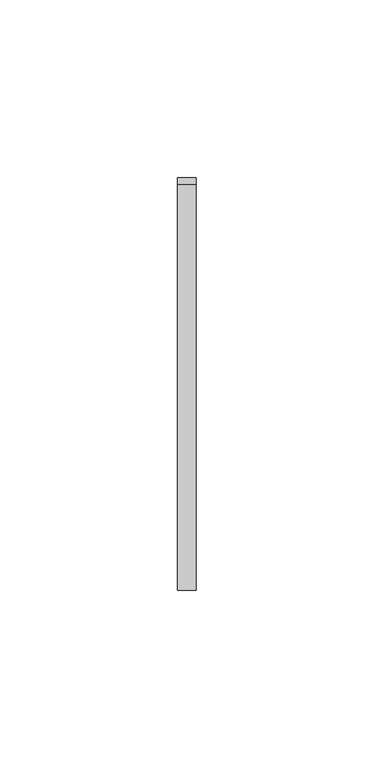
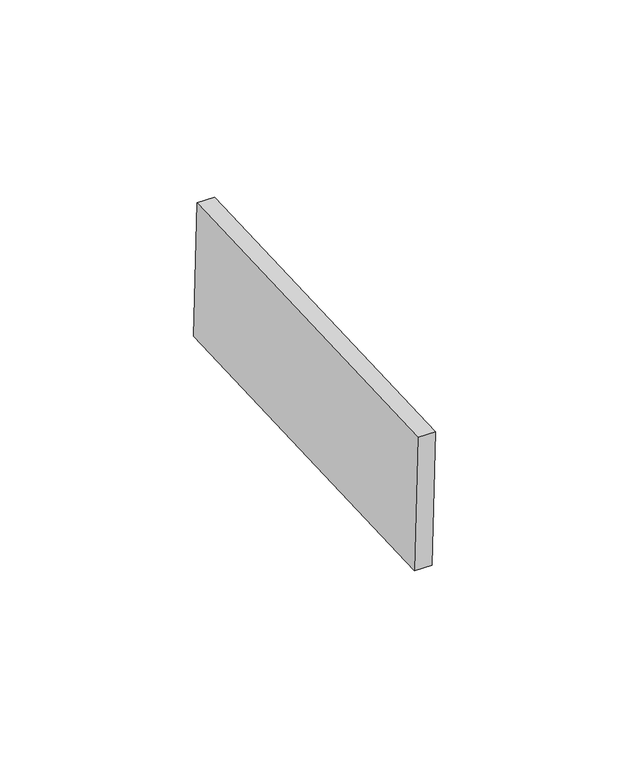
"""IFC4 building model written with IfcOpenShell, lengths in millimetres: proxy geometry, Inner panel:Inner panel:1:Inner panel:1 : Inner panel:Inner panel:300324:2:Inner panel:1:Inner panel:1 : Inner panel:Inner panel:300324:2 : Inner panel:Inner panel:1:Inner panel:1 : Inner panel:Inner panel:300324:300043:100 : Inner panel:Inner panel:1:Inner panel:1 : Inner panel:Inner panel:300324:2:Inner panel:1:Inner panel:1 : Inner panel:Inner panel:300324:2 : Inner panel:Inner panel:1:Inner panel:1 : Inner panel:Inner panel:300324:300043:308120."""

import ifcopenshell
import ifcopenshell.guid

model = None  # the IFC model being written
_history = None  # IfcOwnerHistory: only IFC2X3 demands one
_inside = {}  # id of a spatial element -> (the spatial element, [elements in it])
_under = {}  # id of a project, library or spatial element -> (it, [spatial elements below it])
_declared = {}  # id of a project -> (the project, [libraries it declares])
_typed = {}  # id of a type object -> (the type object, [elements of that type])
_made_of = {}  # id of a material, layer set ... -> (it, [elements and type objects made of it])


def new_model(schema):
    """Start an empty IFC model of exactly this schema.

    Asked for "IFC4X3", IfcOpenShell would pick the latest addendum, in which some entities
    have other attributes; the version numbers below select the first issue.
    IFC2X3 requires an IfcOwnerHistory on every rooted entity: one is made here for all.
    """
    global model, _history
    if schema == "IFC4X3":
        model = ifcopenshell.file(schema_version=(4, 3, 0, 0))
    else:
        model = ifcopenshell.file(schema=schema)
    _inside.clear()
    _under.clear()
    _declared.clear()
    _typed.clear()
    _made_of.clear()
    _history = None
    if model.schema == "IFC2X3":
        org = make("IfcOrganization", Name="unknown")
        user = make(
            "IfcPersonAndOrganization",
            ThePerson=make("IfcPerson", FamilyName="unknown"),
            TheOrganization=org,
        )
        app = make(
            "IfcApplication",
            ApplicationDeveloper=org,
            Version="unknown",
            ApplicationFullName="unknown",
            ApplicationIdentifier="unknown",
        )
        _history = make(
            "IfcOwnerHistory",
            OwningUser=user,
            OwningApplication=app,
            ChangeAction="ADDED",
            CreationDate=0,
        )
    return model


def make(cls, **values):
    """One entity of the class cls with the attributes given. An attribute that is None is left unset."""
    return model.create_entity(
        cls, **{name: value for name, value in values.items() if value is not None}
    )


def rooted(cls, **values):
    """An entity with a GlobalId (a new one), such as an element, a storey or a relation."""
    return make(cls, GlobalId=ifcopenshell.guid.new(), OwnerHistory=_history, **values)


def si_unit(unit_type, name, prefix=None):
    """IfcSIUnit, for example si_unit("LENGTHUNIT", "METRE", prefix="MILLI")."""
    return make("IfcSIUnit", UnitType=unit_type, Prefix=prefix, Name=name)


def assignment(units):
    """IfcUnitAssignment: the units of a project."""
    return None if units is None else make("IfcUnitAssignment", Units=units)


def point(xyz):
    """IfcCartesianPoint."""
    return None if xyz is None else make("IfcCartesianPoint", Coordinates=xyz)


def direction(xyz):
    """IfcDirection."""
    return None if xyz is None else make("IfcDirection", DirectionRatios=xyz)


def frame(location, z_axis=None, x_axis=None):
    """IfcAxis2Placement3D, a coordinate frame: its origin and axes. An axis left out is left unset."""
    return make(
        "IfcAxis2Placement3D",
        Location=point(location),
        Axis=direction(z_axis),
        RefDirection=direction(x_axis),
    )


def origin():
    """The frame at (0, 0, 0) with its axes left unset."""
    return frame((0.0, 0.0, 0.0))


def place(relative_to, where):
    """IfcLocalPlacement: puts the frame where relative to a parent placement (None: the world)."""
    return make(
        "IfcLocalPlacement", PlacementRelTo=relative_to, RelativePlacement=where
    )


def context(
    kind, dimensions, precision=None, world=None, true_north=None, identifier=None
):
    """IfcGeometricRepresentationContext, for example the 3D "Model" context."""
    return make(
        "IfcGeometricRepresentationContext",
        ContextIdentifier=identifier,
        ContextType=kind,
        CoordinateSpaceDimension=dimensions,
        Precision=precision,
        WorldCoordinateSystem=world,
        TrueNorth=true_north,
    )


def project(units=None, contexts=None):
    """IfcProject with its units and contexts."""
    return rooted(
        "IfcProject",
        Name="project",
        RepresentationContexts=contexts,
        UnitsInContext=assignment(units),
    )


def spatial(cls, under=None, at=None, **own):
    """A site, building, storey or space (cls), placed at a placement, below another one or the project."""
    s = rooted(cls, ObjectPlacement=at, **own)
    if under is not None:
        _under.setdefault(under.id(), (under, []))[1].append(s)
    return s


def polyline(points):
    """IfcPolyline through the points."""
    return make("IfcPolyline", Points=[point(p) for p in points])


def outline(outer, holes=None, kind="AREA"):
    """IfcArbitraryClosedProfileDef: a profile drawn as a closed curve; with holes, ...WithVoids."""
    if holes is None:
        return make("IfcArbitraryClosedProfileDef", ProfileType=kind, OuterCurve=outer)
    return make(
        "IfcArbitraryProfileDefWithVoids",
        ProfileType=kind,
        OuterCurve=outer,
        InnerCurves=holes,
    )


def extrude(swept, where, along, depth):
    """IfcExtrudedAreaSolid: the profile swept, set in the frame where, extruded along a direction by depth."""
    return make(
        "IfcExtrudedAreaSolid",
        SweptArea=swept,
        Position=where,
        ExtrudedDirection=direction(along),
        Depth=depth,
    )


def shape(context_of_items, identifier, shape_type, items):
    """IfcShapeRepresentation: the items that make up one representation, for example the "Body"."""
    return make(
        "IfcShapeRepresentation",
        ContextOfItems=context_of_items,
        RepresentationIdentifier=identifier,
        RepresentationType=shape_type,
        Items=items,
    )


def source(mapping_origin, context_of_items, identifier, shape_type, items):
    """IfcRepresentationMap: a shape defined once, which mapped items show again and again."""
    return make(
        "IfcRepresentationMap",
        MappingOrigin=mapping_origin,
        MappedRepresentation=shape(context_of_items, identifier, shape_type, items),
    )


def transform(
    local_origin,
    x_axis=None,
    y_axis=None,
    z_axis=None,
    scale=None,
    scale2=None,
    scale3=None,
    uniform=True,
):
    """IfcCartesianTransformationOperator3D, or its non-uniform kind. x_axis, y_axis, z_axis: its Axis1, 2, 3."""
    if uniform:
        return make(
            "IfcCartesianTransformationOperator3D",
            Axis1=direction(x_axis),
            Axis2=direction(y_axis),
            LocalOrigin=point(local_origin),
            Scale=scale,
            Axis3=direction(z_axis),
        )
    return make(
        "IfcCartesianTransformationOperator3DnonUniform",
        Axis1=direction(x_axis),
        Axis2=direction(y_axis),
        LocalOrigin=point(local_origin),
        Scale=scale,
        Axis3=direction(z_axis),
        Scale2=scale2,
        Scale3=scale3,
    )


def mapped(mapping_source, mapping_target):
    """IfcMappedItem: shows the shape of a source again, moved by a transform."""
    return make(
        "IfcMappedItem", MappingSource=mapping_source, MappingTarget=mapping_target
    )


def made_of(thing, what):
    """Note that an element or type object is made of a material, layer set ...; save() writes the relation."""
    if what is not None:
        _made_of.setdefault(what.id(), (what, []))[1].append(thing)
    return thing


def element(
    cls,
    number,
    at=None,
    inside=None,
    cuts=None,
    type_object=None,
    material=None,
    context=None,
    identifier="Body",
    shape_type=None,
    held_by="IfcProductDefinitionShape",
    body=None,
    shapes=None,
    **own,
):
    """One element of the class cls, such as IfcWall. Its Tag is "e" and its number.

    at: its placement. inside: the storey or other place that contains it. cuts: it is an
    opening in that element (IfcRelVoidsElement). A single representation is given by context,
    identifier, shape_type and body (its items); several are given by shapes. held_by: the class
    of the entity that holds the representations. save() writes the other relations.
    """
    e = rooted(cls, Tag="e%d" % number, ObjectPlacement=at, **own)
    if body is not None:
        shapes = [shape(context, identifier, shape_type, body)]
    if shapes is not None:
        e.Representation = make(held_by, Representations=shapes)
    if inside is not None:
        _inside.setdefault(inside.id(), (inside, []))[1].append(e)
    if cuts is not None:
        rooted(
            "IfcRelVoidsElement", RelatingBuildingElement=cuts, RelatedOpeningElement=e
        )
    if type_object is not None:
        _typed.setdefault(type_object.id(), (type_object, []))[1].append(e)
    return made_of(e, material)


def aggregate(whole, parts):
    """IfcRelAggregates: a whole, such as a stair, and the parts it consists of."""
    return rooted("IfcRelAggregates", RelatingObject=whole, RelatedObjects=parts)


def save(model, path):
    """Write the relations noted so far, then the file.

    IfcRelAggregates (storeys below a building ...), IfcRelContainedInSpatialStructure (elements
    in a storey), IfcRelDefinesByType, IfcRelAssociatesMaterial and IfcRelDeclares: one each for
    every whole, place, type object, material and project.
    """
    for whole, parts in _under.values():
        aggregate(whole, parts)
    for where, things in _inside.values():
        rooted(
            "IfcRelContainedInSpatialStructure",
            RelatedElements=things,
            RelatingStructure=where,
        )
    for kind, things in _typed.values():
        rooted("IfcRelDefinesByType", RelatedObjects=things, RelatingType=kind)
    for what, things in _made_of.values():
        rooted("IfcRelAssociatesMaterial", RelatedObjects=things, RelatingMaterial=what)
    for by, libraries in _declared.values():
        rooted("IfcRelDeclares", RelatingContext=by, RelatedDefinitions=libraries)
    model.write(path)


def generic_models_fb68d92b(model_context):
    return source(origin(), model_context, "Body", "SweptSolid", [
        extrude(outline(polyline([(0.0, -114.3), (0.0, 0.0), (5.2138089, 0.0), (5.2138089, -114.3), (0.0, -114.3)])), frame((591904.595117, -579007.2622385, 3952.103089), z_axis=(0.0, -0.04163054471216399, 0.9991330730923527), x_axis=(-1.0, 0.0, 0.0)), (0.0, 0.0, 1.0), 43.2233908),
    ])


if __name__ == "__main__":
    model = new_model("IFC4")
    model_context = context("Model", 3, world=origin())
    ifc_project = project(units=[si_unit("LENGTHUNIT", "METRE", prefix="MILLI")], contexts=[model_context])
    site = spatial("IfcSite", under=ifc_project)
    building = spatial("IfcBuilding", under=site)
    placement = place(None, origin())
    generic_models_shape = generic_models_fb68d92b(model_context)
    element("IfcBuildingElementProxy", 1, Name="Inner panel:Inner panel:1:Inner panel:1 : Inner panel:Inner panel:300324:2:Inner panel:1:Inner panel:1 : Inner panel:Inner panel:300324:2 : Inner panel:Inner panel:1:Inner panel:1 : Inner panel:Inner panel:300324:300043:100 : Inner panel:Inner panel:1:Inner panel:1 : Inner panel:Inner panel:300324:2:Inner panel:1:Inner panel:1 : Inner panel:Inner panel:300324:2 : Inner panel:Inner panel:1:Inner panel:1 : Inner panel:Inner panel:300324:300043:308120", ObjectType="Inner panel:Inner panel:1:Inner panel:1 : Inner panel:Inner panel:300324:2:Inner panel:1:Inner panel:1 : Inner panel:Inner panel:300324:2 : Inner panel:Inner panel:1:Inner panel:1 : Inner panel:Inner panel:300324:300043:100 : Inner panel:Inner panel:1:Inner panel:1 : Inner panel:Inner panel:300324:2:Inner panel:1:Inner panel:1 : Inner panel:Inner panel:300324:2 : Inner panel:Inner panel:1:Inner panel:1 : Inner panel:Inner panel:300324:300043:308120", at=placement, inside=building, context=model_context, shape_type="MappedRepresentation", body=[
        mapped(generic_models_shape, transform((0.0, 0.0, 0.0), x_axis=(1.0, 0.0, 0.0), y_axis=(0.0, 1.0, 0.0), z_axis=(0.0, 0.0, 1.0))),
    ])
    save(model, "model.ifc")

# Revit data of these elements
# Type "Inner panel:Inner panel:1:Inner panel:1 : Inner panel:Inner panel:300324:2:Inner panel:1:Inner panel:1 : Inner panel:Inner panel:300324:2 : Inner panel:Inner panel:1:Inner panel:1 : Inner panel:Inner panel:300324:300043:100 : Inner panel:Inner panel:1:Inner panel:1 : Inner panel:Inner panel:300324:2:Inner panel:1:Inner panel:1 : Inner panel:Inner panel:300324:2 : Inner panel:Inner panel:1:Inner panel:1 : Inner panel:Inner panel:300324:300043:308120"
#   NameOverride = "Inner panel:Inner panel:1:Inner panel:1 : Inner panel:Inner panel:300324:2:Inner panel:1:Inner panel:1 : Inner panel:Inner panel:300324:2 : Inner panel:Inner panel:1:Inner panel:1 : Inner panel:Inner panel:300324:300043:308120"
#   ObjectTypeOverride = "Inner panel:1:Inner panel:1 : Inner panel:Inner panel:300324:2 : Inner panel:Inner panel:1:Inner panel:1 : Inner panel:Inner panel:300324:300043"
#   Reference = "Inner panel"
#   Tag = "308120"
# Element 1 (IfcBuildingElementProxy, "Inner panel:Inner panel:1:Inner panel:1 : Inner panel:Inner panel:300324:2:Inner panel:1:Inner panel:1 : Inner panel:Inner panel:300324:2 : Inner panel:Inner panel:1:Inner panel:1 : Inner panel:Inner panel:300324:300043:100 : Inner panel:Inner panel:1:Inner panel:1 : Inner panel:Inner panel:300324:2:Inner panel:1:Inner panel:1 : Inner panel:Inner panel:300324:2 : Inner panel:Inner panel:1:Inner panel:1 : Inner panel:Inner panel:300324:300043:308120")
#   Materials on its faces: "SLIDING CLIP"
# Materials
#   "SLIDING CLIP": class "Generic", colour RGB 120 120 120, transparency 0, Cost = 0
